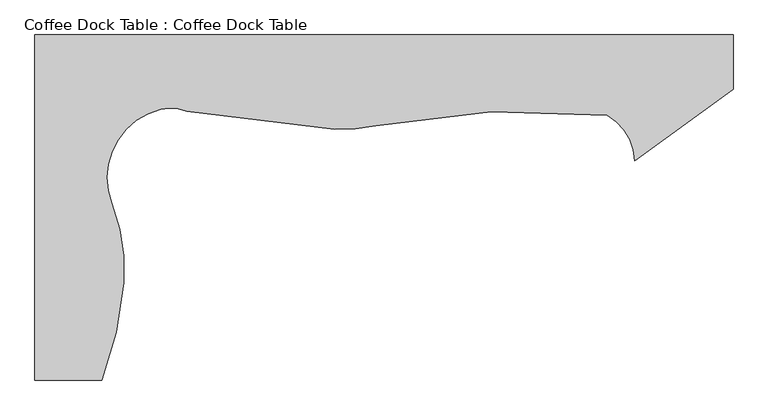
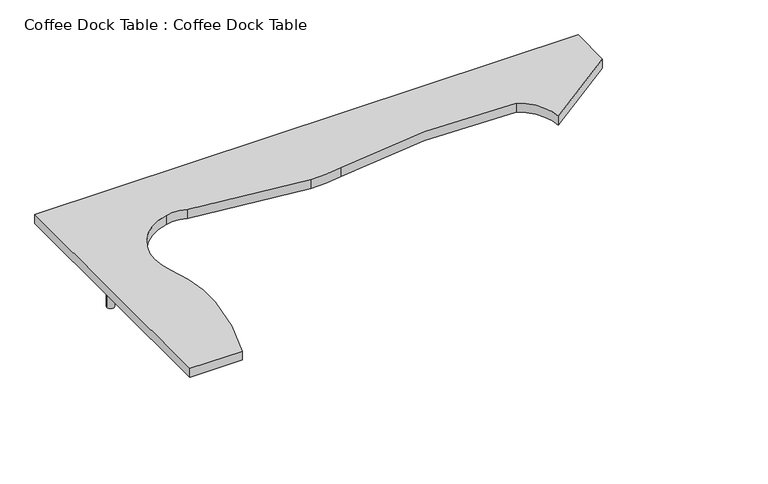
"""IFC4 building model written with IfcOpenShell, lengths in millimetres: furniture geometry, Coffee Dock Table : Coffee Dock Table."""

from ifc_helpers import new_model, si_unit, point, frame, frame_2d, origin, origin_with_axes, place, context, project, spatial, polyline, circle_curve, trimmed, segment, composite_curve, outline, extrude, source, transform, mapped, element, save


def coffee_dock_table_coffee_dock_table_ade3176b(model_context):
    return source(origin(), model_context, "Body", "SweptSolid", [
        extrude(outline(composite_curve([segment(trimmed(circle_curve(frame_2d((6002.9706169, 633.8992416)), 37.5), [point((5965.4706169, 633.8992416))], [point((6040.4706169, 633.8992416))], False, "CARTESIAN"), True, "CONTINUOUS"), segment(trimmed(circle_curve(frame_2d((6002.9706169, 633.8992416)), 37.5), [point((6040.4706169, 633.8992416))], [point((5965.4706169, 633.8992416))], False, "CARTESIAN"), True, "CONTINUOUS")], self_intersect=False)), origin_with_axes(), (0.0, 0.0, 1.0), 800.0),
        extrude(outline(composite_curve([segment(trimmed(circle_curve(frame_2d((3499.9752782, -710.2894555)), 2729.407556), [point((6222.6568816, -901.7848684))], [point((6042.9774794, -1701.6548831))], False, "CARTESIAN"), True, "CONTINUOUS"), segment(polyline([(6042.9774794, -1701.6548831), (5492.9774439, -1701.6548831), (5492.9774439, 1133.7450922), (11228.4774959, 1133.7450922), (11228.4774959, 687.4006799)]), True, "CONTINUOUS"), segment(trimmed(circle_curve(frame_2d((3075.9940033, 11035.7176978)), 13173.8624632), [point((11228.4774959, 687.4006799))], [point((10422.6087077, 100.549451))], False, "CARTESIAN"), True, "CONTINUOUS"), segment(trimmed(circle_curve(frame_2d((9975.8021581, 83.7996648)), 447.1203955), [point((10422.6087077, 100.549451))], [point((10194.4507886, 473.8117473))], True, "CARTESIAN"), True, "CONTINUOUS"), segment(trimmed(circle_curve(frame_2d((9533.8789101, -5847.4497956)), 6355.6827092), [point((10194.4507886, 473.8117473))], [point((8293.0052157, 385.922901))], True, "CARTESIAN"), True, "CONTINUOUS"), segment(trimmed(circle_curve(frame_2d((8000.1475281, 1857.0566048)), 1500.0), [point((8293.0052157, 385.922901))], [point((7956.6428897, 357.687622))], False, "CARTESIAN"), True, "CONTINUOUS"), segment(trimmed(circle_curve(frame_2d((8149.1592486, 6992.6826048)), 6637.7873548), [point((7956.6428897, 357.687622))], [point((6739.7920512, 506.2425125))], False, "CARTESIAN"), True, "CONTINUOUS"), segment(trimmed(circle_curve(frame_2d((6608.4851128, 181.8068672)), 350.0), [point((6739.7920512, 506.2425125))], [point((6525.4609563, 521.8171457))], True, "CARTESIAN"), True, "CONTINUOUS"), segment(trimmed(circle_curve(frame_2d((6662.7550866, -40.4459044)), 578.7827015), [point((6525.4609563, 521.8171457))], [point((6123.6146183, -250.9618683))], True, "CARTESIAN"), True, "CONTINUOUS"), segment(trimmed(circle_curve(frame_2d((4726.3532623, -796.5447702)), 1500.0), [point((6123.6146183, -250.9618683))], [point((6222.6568816, -901.7848684))], False, "CARTESIAN"), True, "CONTINUOUS")], self_intersect=False)), frame((0.0, 0.0, 800.0), z_axis=(0.0, 0.0, 1.0), x_axis=(1.0, 0.0, 0.0)), (0.0, 0.0, 1.0), 100.0),
    ])


if __name__ == "__main__":
    model = new_model("IFC4")
    model_context = context("Model", 3, world=origin())
    ifc_project = project(units=[si_unit("LENGTHUNIT", "METRE", prefix="MILLI")], contexts=[model_context])
    site = spatial("IfcSite", under=ifc_project)
    building = spatial("IfcBuilding", under=site)
    placement = place(None, origin())
    coffee_dock_table_coffee_dock_table_shape = coffee_dock_table_coffee_dock_table_ade3176b(model_context)
    element("IfcFurniture", 1, ObjectType="Coffee Dock Table : Coffee Dock Table", at=placement, inside=building, context=model_context, shape_type="MappedRepresentation", body=[
        mapped(coffee_dock_table_coffee_dock_table_shape, transform((0.0, 0.0, 0.0), x_axis=(1.0, 0.0, 0.0), y_axis=(0.0, 1.0, 0.0), z_axis=(0.0, 0.0, 1.0))),
    ])
    save(model, "model.ifc")

# Revit data of these elements
# Type "Coffee Dock Table : Coffee Dock Table"
#   COBie.Type.CreatedBy = "design@eagle.com"
#   COBie.Type.CreatedOn = "2016-09-13T05:47:35"
#   COBie.Type.Name = "Furniture Systems_Coffee Dock Table_Coffee Dock Table"
#   COBie.Type.Category = "23-40 70 14 64 21 21 : Desk System"
#   COBie.Type.Description = ""
#   COBie.Type.Manufacturer = ""
#   COBie.Type.ModelNumber = ""
#   COBie.Type.ReplacementCost = 0
#   COBie.Type = yes
